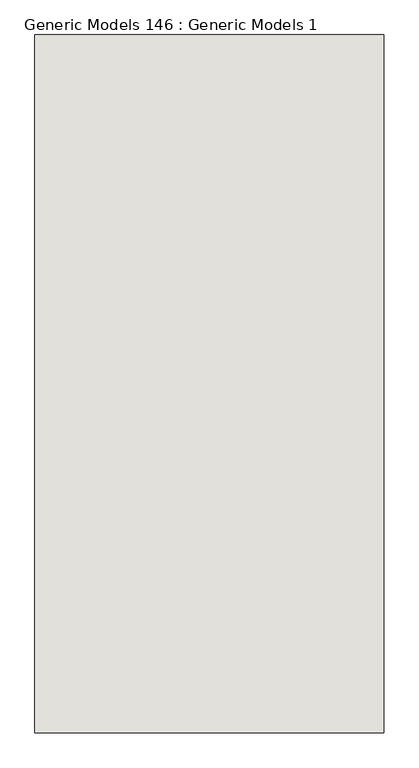
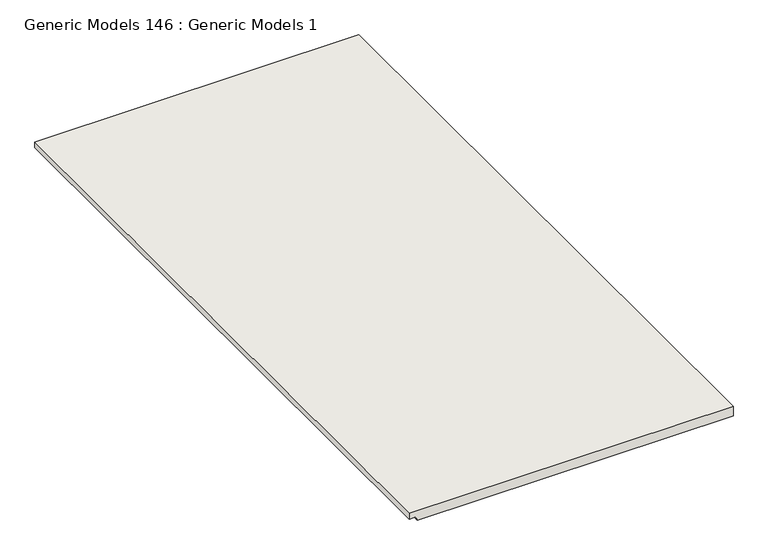
"""IFC4 building model written with IfcOpenShell, lengths in millimetres: wall geometry, Generic Models 146 : Generic Models 1."""

from ifc_helpers import new_model, si_unit, frame, origin, place, context, project, spatial, polyline, outline, extrude, source, transform, mapped, element, save


def generic_models_146_generic_models_1_5c80b7a8(model_context):
    return source(origin(), model_context, "Body", "SweptSolid", [
        extrude(outline(polyline([(1836.9583676, 51016.6701407), (1825.8458676, 51016.6701407), (1825.8458676, 51029.3701407), (1817.9083676, 51032.2591545), (1817.9083676, 51626.2701407), (1836.9583676, 51626.2701407), (1836.9583676, 51016.6701407)])), frame((0.0, 0.0, 0.0), z_axis=(0.0, 1.0, 0.0), x_axis=(0.0, 0.0, 1.0)), (0.0, 0.0, 1.0), 1219.2),
    ])


if __name__ == "__main__":
    model = new_model("IFC4")
    model_context = context("Model", 3, world=origin())
    ifc_project = project(units=[si_unit("LENGTHUNIT", "METRE", prefix="MILLI")], contexts=[model_context])
    site = spatial("IfcSite", under=ifc_project)
    building = spatial("IfcBuilding", under=site)
    placement = place(None, origin())
    generic_models_146_generic_models_1_shape = generic_models_146_generic_models_1_5c80b7a8(model_context)
    element("IfcWall", 1, ObjectType="Generic Models 146 : Generic Models 1", at=placement, inside=building, context=model_context, shape_type="MappedRepresentation", body=[
        mapped(generic_models_146_generic_models_1_shape, transform((0.0, 0.0, 0.0), x_axis=(1.0, 0.0, 0.0), y_axis=(0.0, 1.0, 0.0), z_axis=(0.0, 0.0, 1.0))),
    ])
    save(model, "model.ifc")

# Revit data of these elements
# Element 1 (IfcWall, "Generic Models 146 : Generic Models 1")
#   Materials on its faces: "CEILING AS SCHEDULED"
# Materials
#   "CEILING AS SCHEDULED": class "Generic", colour RGB 255 255 255, transparency 0, Cost = 0
